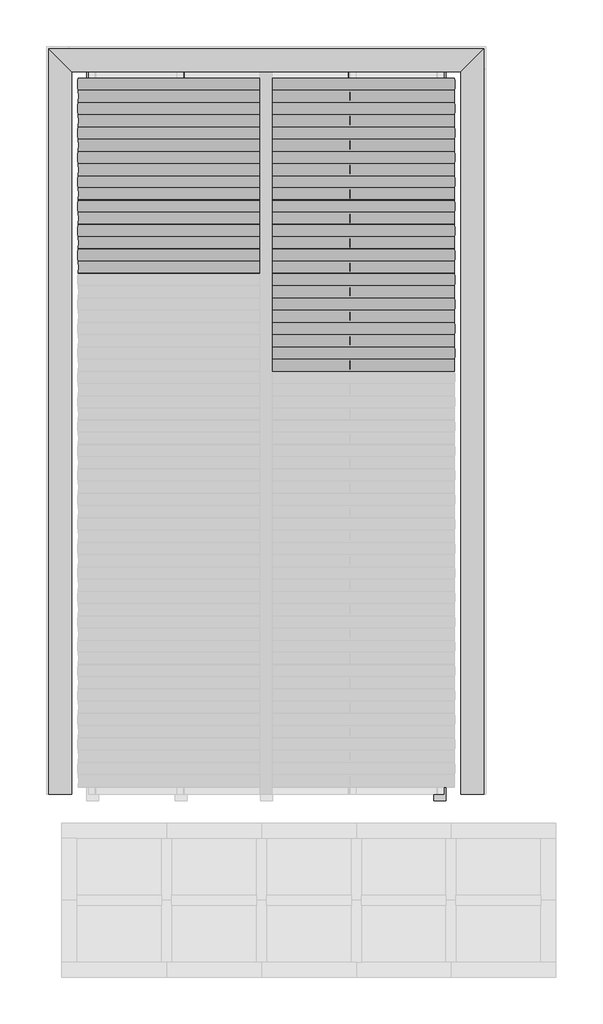
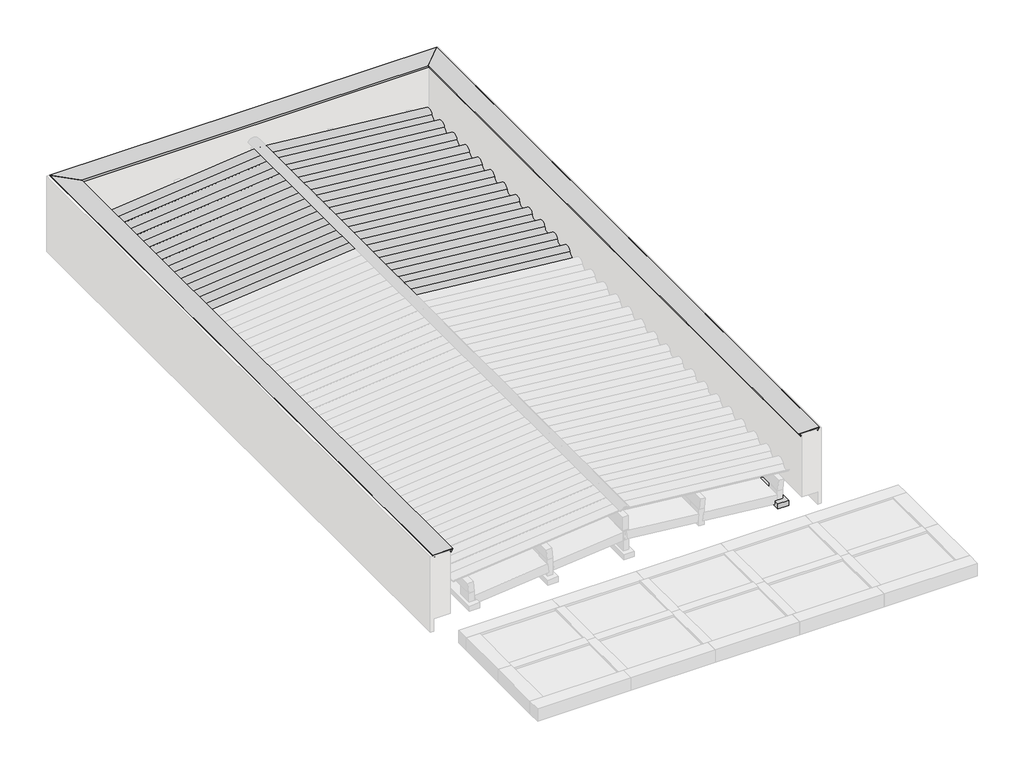
# One storey, part 3 of 3: 33 beams, 12 columns, 1 proxy.
"""IFC4 building model written with IfcOpenShell, lengths in millimetres."""

import ifcopenshell
import ifcopenshell.guid

model = None  # the IFC model being written
_history = None  # IfcOwnerHistory: only IFC2X3 demands one
_inside = {}  # id of a spatial element -> (the spatial element, [elements in it])
_under = {}  # id of a project, library or spatial element -> (it, [spatial elements below it])
_declared = {}  # id of a project -> (the project, [libraries it declares])
_typed = {}  # id of a type object -> (the type object, [elements of that type])
_made_of = {}  # id of a material, layer set ... -> (it, [elements and type objects made of it])


def new_model(schema):
    """Start an empty IFC model of exactly this schema.

    Asked for "IFC4X3", IfcOpenShell would pick the latest addendum, in which some entities
    have other attributes; the version numbers below select the first issue.
    IFC2X3 requires an IfcOwnerHistory on every rooted entity: one is made here for all.
    """
    global model, _history
    if schema == "IFC4X3":
        model = ifcopenshell.file(schema_version=(4, 3, 0, 0))
    else:
        model = ifcopenshell.file(schema=schema)
    _inside.clear()
    _under.clear()
    _declared.clear()
    _typed.clear()
    _made_of.clear()
    _history = None
    if model.schema == "IFC2X3":
        org = make("IfcOrganization", Name="unknown")
        user = make(
            "IfcPersonAndOrganization",
            ThePerson=make("IfcPerson", FamilyName="unknown"),
            TheOrganization=org,
        )
        app = make(
            "IfcApplication",
            ApplicationDeveloper=org,
            Version="unknown",
            ApplicationFullName="unknown",
            ApplicationIdentifier="unknown",
        )
        _history = make(
            "IfcOwnerHistory",
            OwningUser=user,
            OwningApplication=app,
            ChangeAction="ADDED",
            CreationDate=0,
        )
    return model


def make(cls, **values):
    """One entity of the class cls with the attributes given. An attribute that is None is left unset."""
    return model.create_entity(
        cls, **{name: value for name, value in values.items() if value is not None}
    )


def rooted(cls, **values):
    """An entity with a GlobalId (a new one), such as an element, a storey or a relation."""
    return make(cls, GlobalId=ifcopenshell.guid.new(), OwnerHistory=_history, **values)


def si_unit(unit_type, name, prefix=None):
    """IfcSIUnit, for example si_unit("LENGTHUNIT", "METRE", prefix="MILLI")."""
    return make("IfcSIUnit", UnitType=unit_type, Prefix=prefix, Name=name)


def assignment(units):
    """IfcUnitAssignment: the units of a project."""
    return None if units is None else make("IfcUnitAssignment", Units=units)


def point(xyz):
    """IfcCartesianPoint."""
    return None if xyz is None else make("IfcCartesianPoint", Coordinates=xyz)


def direction(xyz):
    """IfcDirection."""
    return None if xyz is None else make("IfcDirection", DirectionRatios=xyz)


def frame(location, z_axis=None, x_axis=None):
    """IfcAxis2Placement3D, a coordinate frame: its origin and axes. An axis left out is left unset."""
    return make(
        "IfcAxis2Placement3D",
        Location=point(location),
        Axis=direction(z_axis),
        RefDirection=direction(x_axis),
    )


def frame_2d(location, x_axis=None):
    """IfcAxis2Placement2D, a coordinate frame in the plane: its origin and x axis."""
    return make(
        "IfcAxis2Placement2D", Location=point(location), RefDirection=direction(x_axis)
    )


def origin():
    """The frame at (0, 0, 0) with its axes left unset."""
    return frame((0.0, 0.0, 0.0))


def place(relative_to, where):
    """IfcLocalPlacement: puts the frame where relative to a parent placement (None: the world)."""
    return make(
        "IfcLocalPlacement", PlacementRelTo=relative_to, RelativePlacement=where
    )


def context(
    kind, dimensions, precision=None, world=None, true_north=None, identifier=None
):
    """IfcGeometricRepresentationContext, for example the 3D "Model" context."""
    return make(
        "IfcGeometricRepresentationContext",
        ContextIdentifier=identifier,
        ContextType=kind,
        CoordinateSpaceDimension=dimensions,
        Precision=precision,
        WorldCoordinateSystem=world,
        TrueNorth=true_north,
    )


def project(units=None, contexts=None):
    """IfcProject with its units and contexts."""
    return rooted(
        "IfcProject",
        Name="project",
        RepresentationContexts=contexts,
        UnitsInContext=assignment(units),
    )


def spatial(cls, under=None, at=None, **own):
    """A site, building, storey or space (cls), placed at a placement, below another one or the project."""
    s = rooted(cls, ObjectPlacement=at, **own)
    if under is not None:
        _under.setdefault(under.id(), (under, []))[1].append(s)
    return s


def polyline(points):
    """IfcPolyline through the points."""
    return make("IfcPolyline", Points=[point(p) for p in points])


def circle_curve(where, radius):
    """IfcCircle in the frame where."""
    return make("IfcCircle", Position=where, Radius=radius)


def trimmed(basis, trim1, trim2, sense, master):
    """IfcTrimmedCurve: the piece of a basis curve between two trims."""
    return make(
        "IfcTrimmedCurve",
        BasisCurve=basis,
        Trim1=trim1,
        Trim2=trim2,
        SenseAgreement=sense,
        MasterRepresentation=master,
    )


def segment(curve, same_sense, transition):
    """IfcCompositeCurveSegment."""
    return make(
        "IfcCompositeCurveSegment",
        Transition=transition,
        SameSense=same_sense,
        ParentCurve=curve,
    )


def composite_curve(segments, self_intersect=None):
    """IfcCompositeCurve: segments joined end to end."""
    return make("IfcCompositeCurve", Segments=segments, SelfIntersect=self_intersect)


def outline(outer, holes=None, kind="AREA"):
    """IfcArbitraryClosedProfileDef: a profile drawn as a closed curve; with holes, ...WithVoids."""
    if holes is None:
        return make("IfcArbitraryClosedProfileDef", ProfileType=kind, OuterCurve=outer)
    return make(
        "IfcArbitraryProfileDefWithVoids",
        ProfileType=kind,
        OuterCurve=outer,
        InnerCurves=holes,
    )


def extrude(swept, where, along, depth):
    """IfcExtrudedAreaSolid: the profile swept, set in the frame where, extruded along a direction by depth."""
    return make(
        "IfcExtrudedAreaSolid",
        SweptArea=swept,
        Position=where,
        ExtrudedDirection=direction(along),
        Depth=depth,
    )


def faces_of(points, faces, orient=None, outer=None):
    """IfcFace entities. A face is a list of loops; a loop is a list of indices into points, from 0.

    orient and outer hold one flag for each loop. By default every Orientation is true, the
    first loop of a face is its IfcFaceOuterBound and the others are IfcFaceBound.
    """
    made = []
    for i, loops in enumerate(faces):
        bounds = []
        for j, loop in enumerate(loops):
            is_outer = j == 0 if outer is None else outer[i][j]
            bounds.append(
                make(
                    "IfcFaceOuterBound" if is_outer else "IfcFaceBound",
                    Bound=make("IfcPolyLoop", Polygon=[points[k] for k in loop]),
                    Orientation=True if orient is None else orient[i][j],
                )
            )
        made.append(make("IfcFace", Bounds=bounds))
    return made


def faceted_brep(points, faces, orient=None, outer=None, voids=None):
    """IfcFacetedBrep: a solid bounded by flat faces; with voids (closed shells), ...WithVoids."""
    shared = [point(p) for p in points]
    hull = make("IfcClosedShell", CfsFaces=faces_of(shared, faces, orient, outer))
    if voids is None:
        return make("IfcFacetedBrep", Outer=hull)
    return make(
        "IfcFacetedBrepWithVoids",
        Outer=hull,
        Voids=[
            make(cls, CfsFaces=faces_of(shared, fs, o, b)) for cls, fs, o, b in voids
        ],
    )


def shape(context_of_items, identifier, shape_type, items):
    """IfcShapeRepresentation: the items that make up one representation, for example the "Body"."""
    return make(
        "IfcShapeRepresentation",
        ContextOfItems=context_of_items,
        RepresentationIdentifier=identifier,
        RepresentationType=shape_type,
        Items=items,
    )


def source(mapping_origin, context_of_items, identifier, shape_type, items):
    """IfcRepresentationMap: a shape defined once, which mapped items show again and again."""
    return make(
        "IfcRepresentationMap",
        MappingOrigin=mapping_origin,
        MappedRepresentation=shape(context_of_items, identifier, shape_type, items),
    )


def transform(
    local_origin,
    x_axis=None,
    y_axis=None,
    z_axis=None,
    scale=None,
    scale2=None,
    scale3=None,
    uniform=True,
):
    """IfcCartesianTransformationOperator3D, or its non-uniform kind. x_axis, y_axis, z_axis: its Axis1, 2, 3."""
    if uniform:
        return make(
            "IfcCartesianTransformationOperator3D",
            Axis1=direction(x_axis),
            Axis2=direction(y_axis),
            LocalOrigin=point(local_origin),
            Scale=scale,
            Axis3=direction(z_axis),
        )
    return make(
        "IfcCartesianTransformationOperator3DnonUniform",
        Axis1=direction(x_axis),
        Axis2=direction(y_axis),
        LocalOrigin=point(local_origin),
        Scale=scale,
        Axis3=direction(z_axis),
        Scale2=scale2,
        Scale3=scale3,
    )


def mapped(mapping_source, mapping_target):
    """IfcMappedItem: shows the shape of a source again, moved by a transform."""
    return make(
        "IfcMappedItem", MappingSource=mapping_source, MappingTarget=mapping_target
    )


def made_of(thing, what):
    """Note that an element or type object is made of a material, layer set ...; save() writes the relation."""
    if what is not None:
        _made_of.setdefault(what.id(), (what, []))[1].append(thing)
    return thing


def element(
    cls,
    number,
    at=None,
    inside=None,
    cuts=None,
    type_object=None,
    material=None,
    context=None,
    identifier="Body",
    shape_type=None,
    held_by="IfcProductDefinitionShape",
    body=None,
    shapes=None,
    **own,
):
    """One element of the class cls, such as IfcWall. Its Tag is "e" and its number.

    at: its placement. inside: the storey or other place that contains it. cuts: it is an
    opening in that element (IfcRelVoidsElement). A single representation is given by context,
    identifier, shape_type and body (its items); several are given by shapes. held_by: the class
    of the entity that holds the representations. save() writes the other relations.
    """
    e = rooted(cls, Tag="e%d" % number, ObjectPlacement=at, **own)
    if body is not None:
        shapes = [shape(context, identifier, shape_type, body)]
    if shapes is not None:
        e.Representation = make(held_by, Representations=shapes)
    if inside is not None:
        _inside.setdefault(inside.id(), (inside, []))[1].append(e)
    if cuts is not None:
        rooted(
            "IfcRelVoidsElement", RelatingBuildingElement=cuts, RelatedOpeningElement=e
        )
    if type_object is not None:
        _typed.setdefault(type_object.id(), (type_object, []))[1].append(e)
    return made_of(e, material)


def aggregate(whole, parts):
    """IfcRelAggregates: a whole, such as a stair, and the parts it consists of."""
    return rooted("IfcRelAggregates", RelatingObject=whole, RelatedObjects=parts)


def save(model, path):
    """Write the relations noted so far, then the file.

    IfcRelAggregates (storeys below a building ...), IfcRelContainedInSpatialStructure (elements
    in a storey), IfcRelDefinesByType, IfcRelAssociatesMaterial and IfcRelDeclares: one each for
    every whole, place, type object, material and project.
    """
    for whole, parts in _under.values():
        aggregate(whole, parts)
    for where, things in _inside.values():
        rooted(
            "IfcRelContainedInSpatialStructure",
            RelatedElements=things,
            RelatingStructure=where,
        )
    for kind, things in _typed.values():
        rooted("IfcRelDefinesByType", RelatedObjects=things, RelatingType=kind)
    for what, things in _made_of.values():
        rooted("IfcRelAssociatesMaterial", RelatedObjects=things, RelatingMaterial=what)
    for by, libraries in _declared.values():
        rooted("IfcRelDeclares", RelatingContext=by, RelatedDefinitions=libraries)
    model.write(path)


def column_1cffec27(model_context):
    return source(origin(), model_context, "Body", "SweptSolid", [
        extrude(outline(polyline([(30.0, 80.0), (30.0, -80.0), (-30.0, -80.0), (-30.0, 80.0), (30.0, 80.0)])), frame((0.0, 0.0, 3110.0), z_axis=(0.0, 0.0, 1.0), x_axis=(1.0, 0.0, 0.0)), (0.0, 0.0, 1.0), 238.0),
    ])


def column_35730ad5(model_context):
    return source(origin(), model_context, "Body", "SweptSolid", [
        extrude(outline(polyline([(30.0, 80.0), (30.0, -80.0), (-30.0, -80.0), (-30.0, 80.0), (30.0, 80.0)])), frame((0.0, 0.0, 3110.0), z_axis=(0.0, 0.0, 1.0), x_axis=(1.0, 0.0, 0.0)), (0.0, 0.0, 1.0), 197.9),
    ])


def column_00c463e4(model_context):
    return source(origin(), model_context, "Body", "SweptSolid", [
        extrude(outline(polyline([(30.0, 80.0), (30.0, -80.0), (-30.0, -80.0), (-30.0, 80.0), (30.0, 80.0)])), frame((0.0, 0.0, 3110.0), z_axis=(0.0, 0.0, 1.0), x_axis=(1.0, 0.0, 0.0)), (0.0, 0.0, 1.0), 109.8),
    ])


model = new_model("IFC4")

# Units and contexts
model_context = context("Model", 3, world=origin())
ifc_project = project(units=[si_unit("LENGTHUNIT", "METRE", prefix="MILLI")], contexts=[model_context])

# Site, building, storey
site = spatial("IfcSite", under=ifc_project)
building = spatial("IfcBuilding", under=site)
storey = spatial("IfcBuildingStorey", under=building, Name="COB. GARAGEM", Elevation=3050.0)

# Beams
placement = place(None, origin())
element("IfcBeam", 1, ObjectType="Madeira de lei : Berço 6x12cm", at=placement, inside=storey, context=model_context, shape_type="SweptSolid", body=[
    extrude(outline(polyline([(-9620.281307, 6423.9300153), (-9500.281307, 6423.9300153), (-9500.281307, 4423.9300153), (-9620.281307, 4423.9300153), (-9620.281307, 6423.9300153)])), frame((0.0, 0.0, 3050.0), z_axis=(0.0, 0.0, 1.0), x_axis=(1.0, 0.0, 0.0)), (0.0, 0.0, 1.0), 60.0),
])
element("IfcBeam", 2, ObjectType="Madeira de lei : Berço 6x12cm", at=placement, inside=storey, context=model_context, shape_type="SweptSolid", body=[
    extrude(outline(polyline([(-9620.281307, 7083.9300153), (-9500.281307, 7083.9300153), (-9500.281307, 6423.9300153), (-9620.281307, 6423.9300153), (-9620.281307, 7083.9300153)])), frame((0.0, 0.0, 3050.0), z_axis=(0.0, 0.0, 1.0), x_axis=(1.0, 0.0, 0.0)), (0.0, 0.0, 1.0), 60.0),
])
element("IfcBeam", 3, ObjectType="Madeira de lei : Berço 6x12cm", at=placement, inside=storey, context=model_context, shape_type="SweptSolid", body=[
    extrude(outline(polyline([(-8767.0824227, 6423.9300153), (-8647.0824227, 6423.9300153), (-8647.0824227, 4423.9300153), (-8767.0824227, 4423.9300153), (-8767.0824227, 6423.9300153)])), frame((0.0, 0.0, 3050.0), z_axis=(0.0, 0.0, 1.0), x_axis=(1.0, 0.0, 0.0)), (0.0, 0.0, 1.0), 60.0),
])
element("IfcBeam", 4, ObjectType="Madeira de lei : Berço 6x12cm", at=placement, inside=storey, context=model_context, shape_type="SweptSolid", body=[
    extrude(outline(polyline([(-8767.0824227, 7083.9300153), (-8647.0824227, 7083.9300153), (-8647.0824227, 6423.9300153), (-8767.0824227, 6423.9300153), (-8767.0824227, 7083.9300153)])), frame((0.0, 0.0, 3050.0), z_axis=(0.0, 0.0, 1.0), x_axis=(1.0, 0.0, 0.0)), (0.0, 0.0, 1.0), 60.0),
])
element("IfcBeam", 5, ObjectType="Madeira de lei : Berço 6x12cm", at=placement, inside=storey, context=model_context, shape_type="SweptSolid", body=[
    extrude(outline(polyline([(-7884.0324227, 4423.9300153), (-7764.0324227, 4423.9300153), (-7764.0324227, 2423.9300153), (-7884.0324227, 2423.9300153), (-7884.0324227, 4423.9300153)])), frame((0.0, 0.0, 3050.0), z_axis=(0.0, 0.0, 1.0), x_axis=(1.0, 0.0, 0.0)), (0.0, 0.0, 1.0), 60.0),
])
element("IfcBeam", 6, ObjectType="Madeira de lei : Berço 6x12cm", at=placement, inside=storey, context=model_context, shape_type="SweptSolid", body=[
    extrude(outline(polyline([(-7884.0324227, 6423.9300153), (-7764.0324227, 6423.9300153), (-7764.0324227, 4423.9300153), (-7884.0324227, 4423.9300153), (-7884.0324227, 6423.9300153)])), frame((0.0, 0.0, 3050.0), z_axis=(0.0, 0.0, 1.0), x_axis=(1.0, 0.0, 0.0)), (0.0, 0.0, 1.0), 60.0),
])
element("IfcBeam", 7, ObjectType="Madeira de lei : Berço 6x12cm", at=placement, inside=storey, context=model_context, shape_type="SweptSolid", body=[
    extrude(outline(polyline([(-7884.0324227, 2423.9300153), (-7764.0324227, 2423.9300153), (-7764.0324227, 423.9300153), (-7884.0324227, 423.9300153), (-7884.0324227, 2423.9300153)])), frame((0.0, 0.0, 3050.0), z_axis=(0.0, 0.0, 1.0), x_axis=(1.0, 0.0, 0.0)), (0.0, 0.0, 1.0), 60.0),
])
element("IfcBeam", 8, ObjectType="Madeira de lei : Berço 6x12cm", at=placement, inside=storey, context=model_context, shape_type="SweptSolid", body=[
    extrude(outline(polyline([(-7884.0324227, 7083.9300153), (-7764.0324227, 7083.9300153), (-7764.0324227, 6423.9300153), (-7884.0324227, 6423.9300153), (-7884.0324227, 7083.9300153)])), frame((0.0, 0.0, 3050.0), z_axis=(0.0, 0.0, 1.0), x_axis=(1.0, 0.0, 0.0)), (0.0, 0.0, 1.0), 60.0),
])
element("IfcBeam", 9, ObjectType="Madeira de lei : Berço 6x12cm", at=placement, inside=storey, context=model_context, shape_type="SweptSolid", body=[
    extrude(outline(polyline([(-7884.0324227, 423.9300153), (-7764.0324227, 423.9300153), (-7764.0324227, -236.0699847), (-7884.0324227, -236.0699847), (-7884.0324227, 423.9300153)])), frame((0.0, 0.0, 3050.0), z_axis=(0.0, 0.0, 1.0), x_axis=(1.0, 0.0, 0.0)), (0.0, 0.0, 1.0), 60.0),
])
element("IfcBeam", 10, ObjectType="Madeira de lei : Berço 6x12cm", at=placement, inside=storey, context=model_context, shape_type="SweptSolid", body=[
    extrude(outline(polyline([(-10473.4801913, 6423.9300153), (-10353.4801913, 6423.9300153), (-10353.4801913, 4423.9300153), (-10473.4801913, 4423.9300153), (-10473.4801913, 6423.9300153)])), frame((0.0, 0.0, 3050.0), z_axis=(0.0, 0.0, 1.0), x_axis=(1.0, 0.0, 0.0)), (0.0, 0.0, 1.0), 60.0),
])
element("IfcBeam", 11, ObjectType="Madeira de lei : Berço 6x12cm", at=placement, inside=storey, context=model_context, shape_type="SweptSolid", body=[
    extrude(outline(polyline([(-10473.4801913, 7083.9300153), (-10353.4801913, 7083.9300153), (-10353.4801913, 6423.9300153), (-10473.4801913, 6423.9300153), (-10473.4801913, 7083.9300153)])), frame((0.0, 0.0, 3050.0), z_axis=(0.0, 0.0, 1.0), x_axis=(1.0, 0.0, 0.0)), (0.0, 0.0, 1.0), 60.0),
])
element("IfcBeam", 12, ObjectType="Madeira de lei : Berço 6x12cm", at=placement, inside=storey, context=model_context, shape_type="SweptSolid", body=[
    extrude(outline(polyline([(-11356.5301913, 6423.9300153), (-11236.5301913, 6423.9300153), (-11236.5301913, 4423.9300153), (-11356.5301913, 4423.9300153), (-11356.5301913, 6423.9300153)])), frame((0.0, 0.0, 3050.0), z_axis=(0.0, 0.0, 1.0), x_axis=(1.0, 0.0, 0.0)), (0.0, 0.0, 1.0), 60.0),
])
element("IfcBeam", 13, ObjectType="Madeira de lei : Berço 6x12cm", at=placement, inside=storey, context=model_context, shape_type="SweptSolid", body=[
    extrude(outline(polyline([(-11356.5301913, 7083.9300153), (-11236.5301913, 7083.9300153), (-11236.5301913, 6423.9300153), (-11356.5301913, 6423.9300153), (-11356.5301913, 7083.9300153)])), frame((0.0, 0.0, 3050.0), z_axis=(0.0, 0.0, 1.0), x_axis=(1.0, 0.0, 0.0)), (0.0, 0.0, 1.0), 60.0),
])
element("IfcBeam", 14, ObjectType="Telha Ondulada : Fibrocimento", at=placement, inside=storey, context=model_context, shape_type="SweptSolid", body=[
    extrude(outline(composite_curve([segment(trimmed(circle_curve(frame_2d((-58.7002979, -53.2060538)), 66.7939461), [point((-29.350149, 6.7939462))], [point((-29.350149, -113.2060538))], False, "CARTESIAN"), True, "CONTINUOUS"), segment(polyline([(-29.350149, -113.2060538), (-31.5472155, -108.7146288)]), True, "CONTINUOUS"), segment(trimmed(circle_curve(frame_2d((-58.7002979, -53.2060538)), 61.7939461), [point((-31.5472155, -108.7146288))], [point((-31.5472155, 2.3025211))], True, "CARTESIAN"), True, "CONTINUOUS"), segment(trimmed(circle_curve(frame_2d((0.0, 66.7939462)), 71.7939461), [point((-31.5472155, 2.3025211))], [point((-31.5472155, 131.2853712))], False, "CARTESIAN"), True, "CONTINUOUS"), segment(polyline([(-31.5472155, 131.2853712), (-29.350149, 126.7939462)]), True, "CONTINUOUS"), segment(trimmed(circle_curve(frame_2d((0.0, 66.7939462)), 66.7939461), [point((-29.350149, 126.7939462))], [point((-29.350149, 6.7939462))], True, "CARTESIAN"), True, "CONTINUOUS")], self_intersect=False)), frame((-11446.918865, 5163.326948, 3394.3067746), z_axis=(0.9950371902099892, 0.0, 0.09950371902099937), x_axis=(-0.09950371902099937, 0.0, 0.9950371902099892)), (0.0, 0.0, 1.0), 1886.8678854),
])
element("IfcBeam", 15, ObjectType="Telha Ondulada : Fibrocimento", at=placement, inside=storey, context=model_context, shape_type="SweptSolid", body=[
    extrude(outline(composite_curve([segment(trimmed(circle_curve(frame_2d((-58.7002979, -53.2060538)), 66.7939461), [point((-29.350149, 6.7939462))], [point((-29.350149, -113.2060538))], False, "CARTESIAN"), True, "CONTINUOUS"), segment(polyline([(-29.350149, -113.2060538), (-31.5472155, -108.7146288)]), True, "CONTINUOUS"), segment(trimmed(circle_curve(frame_2d((-58.7002979, -53.2060538)), 61.7939461), [point((-31.5472155, -108.7146288))], [point((-31.5472155, 2.3025211))], True, "CARTESIAN"), True, "CONTINUOUS"), segment(trimmed(circle_curve(frame_2d((0.0, 66.7939462)), 71.7939461), [point((-31.5472155, 2.3025211))], [point((-31.5472155, 131.2853712))], False, "CARTESIAN"), True, "CONTINUOUS"), segment(polyline([(-31.5472155, 131.2853712), (-29.350149, 126.7939462)]), True, "CONTINUOUS"), segment(trimmed(circle_curve(frame_2d((0.0, 66.7939462)), 66.7939461), [point((-29.350149, 126.7939462))], [point((-29.350149, 6.7939462))], True, "CARTESIAN"), True, "CONTINUOUS")], self_intersect=False)), frame((-11446.918865, 5407.826948, 3394.3067746), z_axis=(0.9950371902099892, 0.0, 0.09950371902099972), x_axis=(-0.09950371902099972, 0.0, 0.9950371902099892)), (0.0, 0.0, 1.0), 1886.8678854),
])
element("IfcBeam", 16, ObjectType="Telha Ondulada : Fibrocimento", at=placement, inside=storey, context=model_context, shape_type="SweptSolid", body=[
    extrude(outline(composite_curve([segment(trimmed(circle_curve(frame_2d((-58.7002979, -53.2060538)), 66.7939461), [point((-29.350149, 6.7939462))], [point((-29.350149, -113.2060538))], False, "CARTESIAN"), True, "CONTINUOUS"), segment(polyline([(-29.350149, -113.2060538), (-31.5472155, -108.7146288)]), True, "CONTINUOUS"), segment(trimmed(circle_curve(frame_2d((-58.7002979, -53.2060538)), 61.7939461), [point((-31.5472155, -108.7146288))], [point((-31.5472155, 2.3025211))], True, "CARTESIAN"), True, "CONTINUOUS"), segment(trimmed(circle_curve(frame_2d((0.0, 66.7939462)), 71.7939461), [point((-31.5472155, 2.3025211))], [point((-31.5472155, 131.2853712))], False, "CARTESIAN"), True, "CONTINUOUS"), segment(polyline([(-31.5472155, 131.2853712), (-29.350149, 126.7939462)]), True, "CONTINUOUS"), segment(trimmed(circle_curve(frame_2d((0.0, 66.7939462)), 66.7939461), [point((-29.350149, 126.7939462))], [point((-29.350149, 6.7939462))], True, "CARTESIAN"), True, "CONTINUOUS")], self_intersect=False)), frame((-11446.918865, 5652.326948, 3394.3067746), z_axis=(0.9950371902099892, 0.0, 0.09950371902099954), x_axis=(-0.09950371902099954, 0.0, 0.9950371902099892)), (0.0, 0.0, 1.0), 1886.8678854),
])
element("IfcBeam", 17, ObjectType="Telha Ondulada : Fibrocimento", at=placement, inside=storey, context=model_context, shape_type="SweptSolid", body=[
    extrude(outline(composite_curve([segment(trimmed(circle_curve(frame_2d((-58.7002979, -53.2060538)), 66.7939461), [point((-29.350149, 6.7939462))], [point((-29.350149, -113.2060538))], False, "CARTESIAN"), True, "CONTINUOUS"), segment(polyline([(-29.350149, -113.2060538), (-31.5472155, -108.7146288)]), True, "CONTINUOUS"), segment(trimmed(circle_curve(frame_2d((-58.7002979, -53.2060538)), 61.7939461), [point((-31.5472155, -108.7146288))], [point((-31.5472155, 2.3025211))], True, "CARTESIAN"), True, "CONTINUOUS"), segment(trimmed(circle_curve(frame_2d((0.0, 66.7939462)), 71.7939461), [point((-31.5472155, 2.3025211))], [point((-31.5472155, 131.2853712))], False, "CARTESIAN"), True, "CONTINUOUS"), segment(polyline([(-31.5472155, 131.2853712), (-29.350149, 126.7939462)]), True, "CONTINUOUS"), segment(trimmed(circle_curve(frame_2d((0.0, 66.7939462)), 66.7939461), [point((-29.350149, 126.7939462))], [point((-29.350149, 6.7939462))], True, "CARTESIAN"), True, "CONTINUOUS")], self_intersect=False)), frame((-11446.918865, 5896.826948, 3394.3067746), z_axis=(0.9950371902099892, 0.0, 0.09950371902099932), x_axis=(-0.09950371902099932, 0.0, 0.9950371902099892)), (0.0, 0.0, 1.0), 1886.8678854),
])
element("IfcBeam", 18, ObjectType="Telha Ondulada : Fibrocimento", at=placement, inside=storey, context=model_context, shape_type="SweptSolid", body=[
    extrude(outline(composite_curve([segment(trimmed(circle_curve(frame_2d((-58.7002979, -53.2060538)), 66.7939461), [point((-29.350149, 6.7939462))], [point((-29.350149, -113.2060538))], False, "CARTESIAN"), True, "CONTINUOUS"), segment(polyline([(-29.350149, -113.2060538), (-31.5472155, -108.7146288)]), True, "CONTINUOUS"), segment(trimmed(circle_curve(frame_2d((-58.7002979, -53.2060538)), 61.7939461), [point((-31.5472155, -108.7146288))], [point((-31.5472155, 2.3025211))], True, "CARTESIAN"), True, "CONTINUOUS"), segment(trimmed(circle_curve(frame_2d((0.0, 66.7939462)), 71.7939461), [point((-31.5472155, 2.3025211))], [point((-31.5472155, 131.2853712))], False, "CARTESIAN"), True, "CONTINUOUS"), segment(polyline([(-31.5472155, 131.2853712), (-29.350149, 126.7939462)]), True, "CONTINUOUS"), segment(trimmed(circle_curve(frame_2d((0.0, 66.7939462)), 66.7939461), [point((-29.350149, 126.7939462))], [point((-29.350149, 6.7939462))], True, "CARTESIAN"), True, "CONTINUOUS")], self_intersect=False)), frame((-11446.918865, 6141.326948, 3394.3067746), z_axis=(0.9950371902099892, 0.0, 0.09950371902099943), x_axis=(-0.09950371902099943, 0.0, 0.9950371902099892)), (0.0, 0.0, 1.0), 1886.8678854),
])
element("IfcBeam", 19, ObjectType="Telha Ondulada : Fibrocimento", at=placement, inside=storey, context=model_context, shape_type="SweptSolid", body=[
    extrude(outline(composite_curve([segment(trimmed(circle_curve(frame_2d((-58.7002979, -53.2060538)), 66.7939461), [point((-29.350149, 6.7939462))], [point((-29.350149, -113.2060538))], False, "CARTESIAN"), True, "CONTINUOUS"), segment(polyline([(-29.350149, -113.2060538), (-31.5472155, -108.7146288)]), True, "CONTINUOUS"), segment(trimmed(circle_curve(frame_2d((-58.7002979, -53.2060538)), 61.7939461), [point((-31.5472155, -108.7146288))], [point((-31.5472155, 2.3025211))], True, "CARTESIAN"), True, "CONTINUOUS"), segment(trimmed(circle_curve(frame_2d((0.0, 66.7939462)), 71.7939461), [point((-31.5472155, 2.3025211))], [point((-31.5472155, 131.2853712))], False, "CARTESIAN"), True, "CONTINUOUS"), segment(polyline([(-31.5472155, 131.2853712), (-29.350149, 126.7939462)]), True, "CONTINUOUS"), segment(trimmed(circle_curve(frame_2d((0.0, 66.7939462)), 66.7939461), [point((-29.350149, 126.7939462))], [point((-29.350149, 6.7939462))], True, "CARTESIAN"), True, "CONTINUOUS")], self_intersect=False)), frame((-11446.918865, 6385.826948, 3394.3067746), z_axis=(0.9950371902099892, 0.0, 0.09950371902099919), x_axis=(-0.09950371902099919, 0.0, 0.9950371902099892)), (0.0, 0.0, 1.0), 1886.8678854),
])
element("IfcBeam", 20, ObjectType="Telha Ondulada : Fibrocimento", at=placement, inside=storey, context=model_context, shape_type="SweptSolid", body=[
    extrude(outline(composite_curve([segment(trimmed(circle_curve(frame_2d((-58.7002979, -53.2060538)), 66.7939461), [point((-29.350149, 6.7939462))], [point((-29.350149, -113.2060538))], False, "CARTESIAN"), True, "CONTINUOUS"), segment(polyline([(-29.350149, -113.2060538), (-31.5472155, -108.7146288)]), True, "CONTINUOUS"), segment(trimmed(circle_curve(frame_2d((-58.7002979, -53.2060538)), 61.7939461), [point((-31.5472155, -108.7146288))], [point((-31.5472155, 2.3025211))], True, "CARTESIAN"), True, "CONTINUOUS"), segment(trimmed(circle_curve(frame_2d((0.0, 66.7939462)), 71.7939461), [point((-31.5472155, 2.3025211))], [point((-31.5472155, 131.2853712))], False, "CARTESIAN"), True, "CONTINUOUS"), segment(polyline([(-31.5472155, 131.2853712), (-29.350149, 126.7939462)]), True, "CONTINUOUS"), segment(trimmed(circle_curve(frame_2d((0.0, 66.7939462)), 66.7939461), [point((-29.350149, 126.7939462))], [point((-29.350149, 6.7939462))], True, "CARTESIAN"), True, "CONTINUOUS")], self_intersect=False)), frame((-11446.918865, 6630.326948, 3394.3067746), z_axis=(0.9950371902099892, 0.0, 0.09950371902099925), x_axis=(-0.09950371902099925, 0.0, 0.9950371902099892)), (0.0, 0.0, 1.0), 1886.8678854),
])
element("IfcBeam", 21, ObjectType="Telha Ondulada : Fibrocimento", at=placement, inside=storey, context=model_context, shape_type="SweptSolid", body=[
    extrude(outline(composite_curve([segment(trimmed(circle_curve(frame_2d((-58.7002979, -53.2060538)), 66.7939461), [point((-29.350149, 6.7939462))], [point((-29.350149, -113.2060538))], False, "CARTESIAN"), True, "CONTINUOUS"), segment(polyline([(-29.350149, -113.2060538), (-31.5472155, -108.7146288)]), True, "CONTINUOUS"), segment(trimmed(circle_curve(frame_2d((-58.7002979, -53.2060538)), 61.7939461), [point((-31.5472155, -108.7146288))], [point((-31.5472155, 2.3025211))], True, "CARTESIAN"), True, "CONTINUOUS"), segment(trimmed(circle_curve(frame_2d((0.0, 66.7939462)), 71.7939461), [point((-31.5472155, 2.3025211))], [point((-31.5472155, 131.2853712))], False, "CARTESIAN"), True, "CONTINUOUS"), segment(polyline([(-31.5472155, 131.2853712), (-29.350149, 126.7939462)]), True, "CONTINUOUS"), segment(trimmed(circle_curve(frame_2d((0.0, 66.7939462)), 66.7939461), [point((-29.350149, 126.7939462))], [point((-29.350149, 6.7939462))], True, "CARTESIAN"), True, "CONTINUOUS")], self_intersect=False)), frame((-11446.918865, 6874.826948, 3394.3067746), z_axis=(0.9950371902099892, 0.0, 0.09950371902099937), x_axis=(-0.09950371902099937, 0.0, 0.9950371902099892)), (0.0, 0.0, 1.0), 1886.8678854),
])
element("IfcBeam", 22, ObjectType="Telha Ondulada : Fibrocimento", at=placement, inside=storey, context=model_context, shape_type="SweptSolid", body=[
    extrude(outline(composite_curve([segment(trimmed(circle_curve(frame_2d((0.0, 66.7939462)), 66.7939461), [point((29.350149, 6.7939462))], [point((29.350149, 126.7939462))], True, "CARTESIAN"), True, "CONTINUOUS"), segment(polyline([(29.350149, 126.7939462), (31.5472155, 131.2853712)]), True, "CONTINUOUS"), segment(trimmed(circle_curve(frame_2d((0.0, 66.7939462)), 71.7939461), [point((31.5472155, 131.2853712))], [point((31.5472155, 2.3025211))], False, "CARTESIAN"), True, "CONTINUOUS"), segment(trimmed(circle_curve(frame_2d((58.7002979, -53.2060538)), 61.7939461), [point((31.5472155, 2.3025211))], [point((31.5472155, -108.7146288))], True, "CARTESIAN"), True, "CONTINUOUS"), segment(polyline([(31.5472155, -108.7146288), (29.350149, -113.2060538)]), True, "CONTINUOUS"), segment(trimmed(circle_curve(frame_2d((58.7002979, -53.2060538)), 66.7939461), [point((29.350149, -113.2060538))], [point((29.350149, 6.7939462))], False, "CARTESIAN"), True, "CONTINUOUS")], self_intersect=False)), frame((-7673.6437489, 4185.326948, 3394.3067746), z_axis=(-0.9950371902099892, 0.0, 0.09950371902099965), x_axis=(-0.09950371902099965, 0.0, -0.9950371902099892)), (0.0, 0.0, 1.0), 1886.8678854),
])
element("IfcBeam", 23, ObjectType="Telha Ondulada : Fibrocimento", at=placement, inside=storey, context=model_context, shape_type="SweptSolid", body=[
    extrude(outline(composite_curve([segment(trimmed(circle_curve(frame_2d((0.0, 66.7939462)), 66.7939461), [point((29.350149, 6.7939462))], [point((29.350149, 126.7939462))], True, "CARTESIAN"), True, "CONTINUOUS"), segment(polyline([(29.350149, 126.7939462), (31.5472155, 131.2853712)]), True, "CONTINUOUS"), segment(trimmed(circle_curve(frame_2d((0.0, 66.7939462)), 71.7939461), [point((31.5472155, 131.2853712))], [point((31.5472155, 2.3025211))], False, "CARTESIAN"), True, "CONTINUOUS"), segment(trimmed(circle_curve(frame_2d((58.7002979, -53.2060538)), 61.7939461), [point((31.5472155, 2.3025211))], [point((31.5472155, -108.7146288))], True, "CARTESIAN"), True, "CONTINUOUS"), segment(polyline([(31.5472155, -108.7146288), (29.350149, -113.2060538)]), True, "CONTINUOUS"), segment(trimmed(circle_curve(frame_2d((58.7002979, -53.2060538)), 66.7939461), [point((29.350149, -113.2060538))], [point((29.350149, 6.7939462))], False, "CARTESIAN"), True, "CONTINUOUS")], self_intersect=False)), frame((-7673.6437489, 4429.826948, 3394.3067746), z_axis=(-0.9950371902099892, 0.0, 0.09950371902099965), x_axis=(-0.09950371902099965, 0.0, -0.9950371902099892)), (0.0, 0.0, 1.0), 1886.8678854),
])
element("IfcBeam", 24, ObjectType="Telha Ondulada : Fibrocimento", at=placement, inside=storey, context=model_context, shape_type="SweptSolid", body=[
    extrude(outline(composite_curve([segment(trimmed(circle_curve(frame_2d((0.0, 66.7939462)), 66.7939461), [point((29.350149, 6.7939462))], [point((29.350149, 126.7939462))], True, "CARTESIAN"), True, "CONTINUOUS"), segment(polyline([(29.350149, 126.7939462), (31.5472155, 131.2853712)]), True, "CONTINUOUS"), segment(trimmed(circle_curve(frame_2d((0.0, 66.7939462)), 71.7939461), [point((31.5472155, 131.2853712))], [point((31.5472155, 2.3025211))], False, "CARTESIAN"), True, "CONTINUOUS"), segment(trimmed(circle_curve(frame_2d((58.7002979, -53.2060538)), 61.7939461), [point((31.5472155, 2.3025211))], [point((31.5472155, -108.7146288))], True, "CARTESIAN"), True, "CONTINUOUS"), segment(polyline([(31.5472155, -108.7146288), (29.350149, -113.2060538)]), True, "CONTINUOUS"), segment(trimmed(circle_curve(frame_2d((58.7002979, -53.2060538)), 66.7939461), [point((29.350149, -113.2060538))], [point((29.350149, 6.7939462))], False, "CARTESIAN"), True, "CONTINUOUS")], self_intersect=False)), frame((-7673.6437489, 4674.326948, 3394.3067746), z_axis=(-0.9950371902099892, 0.0, 0.09950371902099965), x_axis=(-0.09950371902099965, 0.0, -0.9950371902099892)), (0.0, 0.0, 1.0), 1886.8678854),
])
element("IfcBeam", 25, ObjectType="Telha Ondulada : Fibrocimento", at=placement, inside=storey, context=model_context, shape_type="SweptSolid", body=[
    extrude(outline(composite_curve([segment(trimmed(circle_curve(frame_2d((0.0, 66.7939462)), 66.7939461), [point((29.350149, 6.7939462))], [point((29.350149, 126.7939462))], True, "CARTESIAN"), True, "CONTINUOUS"), segment(polyline([(29.350149, 126.7939462), (31.5472155, 131.2853712)]), True, "CONTINUOUS"), segment(trimmed(circle_curve(frame_2d((0.0, 66.7939462)), 71.7939461), [point((31.5472155, 131.2853712))], [point((31.5472155, 2.3025211))], False, "CARTESIAN"), True, "CONTINUOUS"), segment(trimmed(circle_curve(frame_2d((58.7002979, -53.2060538)), 61.7939461), [point((31.5472155, 2.3025211))], [point((31.5472155, -108.7146288))], True, "CARTESIAN"), True, "CONTINUOUS"), segment(polyline([(31.5472155, -108.7146288), (29.350149, -113.2060538)]), True, "CONTINUOUS"), segment(trimmed(circle_curve(frame_2d((58.7002979, -53.2060538)), 66.7939461), [point((29.350149, -113.2060538))], [point((29.350149, 6.7939462))], False, "CARTESIAN"), True, "CONTINUOUS")], self_intersect=False)), frame((-7673.6437489, 4918.826948, 3394.3067746), z_axis=(-0.9950371902099892, 0.0, 0.09950371902099965), x_axis=(-0.09950371902099965, 0.0, -0.9950371902099892)), (0.0, 0.0, 1.0), 1886.8678854),
])
element("IfcBeam", 26, ObjectType="Telha Ondulada : Fibrocimento", at=placement, inside=storey, context=model_context, shape_type="SweptSolid", body=[
    extrude(outline(composite_curve([segment(trimmed(circle_curve(frame_2d((0.0, 66.7939462)), 66.7939461), [point((29.350149, 6.7939462))], [point((29.350149, 126.7939462))], True, "CARTESIAN"), True, "CONTINUOUS"), segment(polyline([(29.350149, 126.7939462), (31.5472155, 131.2853712)]), True, "CONTINUOUS"), segment(trimmed(circle_curve(frame_2d((0.0, 66.7939462)), 71.7939461), [point((31.5472155, 131.2853712))], [point((31.5472155, 2.3025211))], False, "CARTESIAN"), True, "CONTINUOUS"), segment(trimmed(circle_curve(frame_2d((58.7002979, -53.2060538)), 61.7939461), [point((31.5472155, 2.3025211))], [point((31.5472155, -108.7146288))], True, "CARTESIAN"), True, "CONTINUOUS"), segment(polyline([(31.5472155, -108.7146288), (29.350149, -113.2060538)]), True, "CONTINUOUS"), segment(trimmed(circle_curve(frame_2d((58.7002979, -53.2060538)), 66.7939461), [point((29.350149, -113.2060538))], [point((29.350149, 6.7939462))], False, "CARTESIAN"), True, "CONTINUOUS")], self_intersect=False)), frame((-7673.6437489, 5163.326948, 3394.3067746), z_axis=(-0.9950371902099892, 0.0, 0.09950371902099965), x_axis=(-0.09950371902099965, 0.0, -0.9950371902099892)), (0.0, 0.0, 1.0), 1886.8678854),
])
element("IfcBeam", 27, ObjectType="Telha Ondulada : Fibrocimento", at=placement, inside=storey, context=model_context, shape_type="SweptSolid", body=[
    extrude(outline(composite_curve([segment(trimmed(circle_curve(frame_2d((0.0, 66.7939462)), 66.7939461), [point((29.350149, 6.7939462))], [point((29.350149, 126.7939462))], True, "CARTESIAN"), True, "CONTINUOUS"), segment(polyline([(29.350149, 126.7939462), (31.5472155, 131.2853712)]), True, "CONTINUOUS"), segment(trimmed(circle_curve(frame_2d((0.0, 66.7939462)), 71.7939461), [point((31.5472155, 131.2853712))], [point((31.5472155, 2.3025211))], False, "CARTESIAN"), True, "CONTINUOUS"), segment(trimmed(circle_curve(frame_2d((58.7002979, -53.2060538)), 61.7939461), [point((31.5472155, 2.3025211))], [point((31.5472155, -108.7146288))], True, "CARTESIAN"), True, "CONTINUOUS"), segment(polyline([(31.5472155, -108.7146288), (29.350149, -113.2060538)]), True, "CONTINUOUS"), segment(trimmed(circle_curve(frame_2d((58.7002979, -53.2060538)), 66.7939461), [point((29.350149, -113.2060538))], [point((29.350149, 6.7939462))], False, "CARTESIAN"), True, "CONTINUOUS")], self_intersect=False)), frame((-7673.6437489, 5407.826948, 3394.3067746), z_axis=(-0.9950371902099892, 0.0, 0.09950371902099965), x_axis=(-0.09950371902099965, 0.0, -0.9950371902099892)), (0.0, 0.0, 1.0), 1886.8678854),
])
element("IfcBeam", 28, ObjectType="Telha Ondulada : Fibrocimento", at=placement, inside=storey, context=model_context, shape_type="SweptSolid", body=[
    extrude(outline(composite_curve([segment(trimmed(circle_curve(frame_2d((0.0, 66.7939462)), 66.7939461), [point((29.350149, 6.7939462))], [point((29.350149, 126.7939462))], True, "CARTESIAN"), True, "CONTINUOUS"), segment(polyline([(29.350149, 126.7939462), (31.5472155, 131.2853712)]), True, "CONTINUOUS"), segment(trimmed(circle_curve(frame_2d((0.0, 66.7939462)), 71.7939461), [point((31.5472155, 131.2853712))], [point((31.5472155, 2.3025211))], False, "CARTESIAN"), True, "CONTINUOUS"), segment(trimmed(circle_curve(frame_2d((58.7002979, -53.2060538)), 61.7939461), [point((31.5472155, 2.3025211))], [point((31.5472155, -108.7146288))], True, "CARTESIAN"), True, "CONTINUOUS"), segment(polyline([(31.5472155, -108.7146288), (29.350149, -113.2060538)]), True, "CONTINUOUS"), segment(trimmed(circle_curve(frame_2d((58.7002979, -53.2060538)), 66.7939461), [point((29.350149, -113.2060538))], [point((29.350149, 6.7939462))], False, "CARTESIAN"), True, "CONTINUOUS")], self_intersect=False)), frame((-7673.6437489, 5652.326948, 3394.3067746), z_axis=(-0.9950371902099892, 0.0, 0.09950371902099965), x_axis=(-0.09950371902099965, 0.0, -0.9950371902099892)), (0.0, 0.0, 1.0), 1886.8678854),
])
element("IfcBeam", 29, ObjectType="Telha Ondulada : Fibrocimento", at=placement, inside=storey, context=model_context, shape_type="SweptSolid", body=[
    extrude(outline(composite_curve([segment(trimmed(circle_curve(frame_2d((0.0, 66.7939462)), 66.7939461), [point((29.350149, 6.7939462))], [point((29.350149, 126.7939462))], True, "CARTESIAN"), True, "CONTINUOUS"), segment(polyline([(29.350149, 126.7939462), (31.5472155, 131.2853712)]), True, "CONTINUOUS"), segment(trimmed(circle_curve(frame_2d((0.0, 66.7939462)), 71.7939461), [point((31.5472155, 131.2853712))], [point((31.5472155, 2.3025211))], False, "CARTESIAN"), True, "CONTINUOUS"), segment(trimmed(circle_curve(frame_2d((58.7002979, -53.2060538)), 61.7939461), [point((31.5472155, 2.3025211))], [point((31.5472155, -108.7146288))], True, "CARTESIAN"), True, "CONTINUOUS"), segment(polyline([(31.5472155, -108.7146288), (29.350149, -113.2060538)]), True, "CONTINUOUS"), segment(trimmed(circle_curve(frame_2d((58.7002979, -53.2060538)), 66.7939461), [point((29.350149, -113.2060538))], [point((29.350149, 6.7939462))], False, "CARTESIAN"), True, "CONTINUOUS")], self_intersect=False)), frame((-7673.6437489, 5896.826948, 3394.3067746), z_axis=(-0.9950371902099892, 0.0, 0.09950371902099965), x_axis=(-0.09950371902099965, 0.0, -0.9950371902099892)), (0.0, 0.0, 1.0), 1886.8678854),
])
element("IfcBeam", 30, ObjectType="Telha Ondulada : Fibrocimento", at=placement, inside=storey, context=model_context, shape_type="SweptSolid", body=[
    extrude(outline(composite_curve([segment(trimmed(circle_curve(frame_2d((0.0, 66.7939462)), 66.7939461), [point((29.350149, 6.7939462))], [point((29.350149, 126.7939462))], True, "CARTESIAN"), True, "CONTINUOUS"), segment(polyline([(29.350149, 126.7939462), (31.5472155, 131.2853712)]), True, "CONTINUOUS"), segment(trimmed(circle_curve(frame_2d((0.0, 66.7939462)), 71.7939461), [point((31.5472155, 131.2853712))], [point((31.5472155, 2.3025211))], False, "CARTESIAN"), True, "CONTINUOUS"), segment(trimmed(circle_curve(frame_2d((58.7002979, -53.2060538)), 61.7939461), [point((31.5472155, 2.3025211))], [point((31.5472155, -108.7146288))], True, "CARTESIAN"), True, "CONTINUOUS"), segment(polyline([(31.5472155, -108.7146288), (29.350149, -113.2060538)]), True, "CONTINUOUS"), segment(trimmed(circle_curve(frame_2d((58.7002979, -53.2060538)), 66.7939461), [point((29.350149, -113.2060538))], [point((29.350149, 6.7939462))], False, "CARTESIAN"), True, "CONTINUOUS")], self_intersect=False)), frame((-7673.6437489, 6141.326948, 3394.3067746), z_axis=(-0.9950371902099892, 0.0, 0.09950371902099965), x_axis=(-0.09950371902099965, 0.0, -0.9950371902099892)), (0.0, 0.0, 1.0), 1886.8678854),
])
element("IfcBeam", 31, ObjectType="Telha Ondulada : Fibrocimento", at=placement, inside=storey, context=model_context, shape_type="SweptSolid", body=[
    extrude(outline(composite_curve([segment(trimmed(circle_curve(frame_2d((0.0, 66.7939462)), 66.7939461), [point((29.350149, 6.7939462))], [point((29.350149, 126.7939462))], True, "CARTESIAN"), True, "CONTINUOUS"), segment(polyline([(29.350149, 126.7939462), (31.5472155, 131.2853712)]), True, "CONTINUOUS"), segment(trimmed(circle_curve(frame_2d((0.0, 66.7939462)), 71.7939461), [point((31.5472155, 131.2853712))], [point((31.5472155, 2.3025211))], False, "CARTESIAN"), True, "CONTINUOUS"), segment(trimmed(circle_curve(frame_2d((58.7002979, -53.2060538)), 61.7939461), [point((31.5472155, 2.3025211))], [point((31.5472155, -108.7146288))], True, "CARTESIAN"), True, "CONTINUOUS"), segment(polyline([(31.5472155, -108.7146288), (29.350149, -113.2060538)]), True, "CONTINUOUS"), segment(trimmed(circle_curve(frame_2d((58.7002979, -53.2060538)), 66.7939461), [point((29.350149, -113.2060538))], [point((29.350149, 6.7939462))], False, "CARTESIAN"), True, "CONTINUOUS")], self_intersect=False)), frame((-7673.6437489, 6385.826948, 3394.3067746), z_axis=(-0.9950371902099892, 0.0, 0.09950371902099965), x_axis=(-0.09950371902099965, 0.0, -0.9950371902099892)), (0.0, 0.0, 1.0), 1886.8678854),
])
element("IfcBeam", 32, ObjectType="Telha Ondulada : Fibrocimento", at=placement, inside=storey, context=model_context, shape_type="SweptSolid", body=[
    extrude(outline(composite_curve([segment(trimmed(circle_curve(frame_2d((0.0, 66.7939462)), 66.7939461), [point((29.350149, 6.7939462))], [point((29.350149, 126.7939462))], True, "CARTESIAN"), True, "CONTINUOUS"), segment(polyline([(29.350149, 126.7939462), (31.5472155, 131.2853712)]), True, "CONTINUOUS"), segment(trimmed(circle_curve(frame_2d((0.0, 66.7939462)), 71.7939461), [point((31.5472155, 131.2853712))], [point((31.5472155, 2.3025211))], False, "CARTESIAN"), True, "CONTINUOUS"), segment(trimmed(circle_curve(frame_2d((58.7002979, -53.2060538)), 61.7939461), [point((31.5472155, 2.3025211))], [point((31.5472155, -108.7146288))], True, "CARTESIAN"), True, "CONTINUOUS"), segment(polyline([(31.5472155, -108.7146288), (29.350149, -113.2060538)]), True, "CONTINUOUS"), segment(trimmed(circle_curve(frame_2d((58.7002979, -53.2060538)), 66.7939461), [point((29.350149, -113.2060538))], [point((29.350149, 6.7939462))], False, "CARTESIAN"), True, "CONTINUOUS")], self_intersect=False)), frame((-7673.6437489, 6630.326948, 3394.3067746), z_axis=(-0.9950371902099892, 0.0, 0.09950371902099965), x_axis=(-0.09950371902099965, 0.0, -0.9950371902099892)), (0.0, 0.0, 1.0), 1886.8678854),
])
element("IfcBeam", 33, ObjectType="Telha Ondulada : Fibrocimento", at=placement, inside=storey, context=model_context, shape_type="SweptSolid", body=[
    extrude(outline(composite_curve([segment(trimmed(circle_curve(frame_2d((0.0, 66.7939462)), 66.7939461), [point((29.350149, 6.7939462))], [point((29.350149, 126.7939462))], True, "CARTESIAN"), True, "CONTINUOUS"), segment(polyline([(29.350149, 126.7939462), (31.5472155, 131.2853712)]), True, "CONTINUOUS"), segment(trimmed(circle_curve(frame_2d((0.0, 66.7939462)), 71.7939461), [point((31.5472155, 131.2853712))], [point((31.5472155, 2.3025211))], False, "CARTESIAN"), True, "CONTINUOUS"), segment(trimmed(circle_curve(frame_2d((58.7002979, -53.2060538)), 61.7939461), [point((31.5472155, 2.3025211))], [point((31.5472155, -108.7146288))], True, "CARTESIAN"), True, "CONTINUOUS"), segment(polyline([(31.5472155, -108.7146288), (29.350149, -113.2060538)]), True, "CONTINUOUS"), segment(trimmed(circle_curve(frame_2d((58.7002979, -53.2060538)), 66.7939461), [point((29.350149, -113.2060538))], [point((29.350149, 6.7939462))], False, "CARTESIAN"), True, "CONTINUOUS")], self_intersect=False)), frame((-7673.6437489, 6874.826948, 3394.3067746), z_axis=(-0.9950371902099892, 0.0, 0.09950371902099965), x_axis=(-0.09950371902099965, 0.0, -0.9950371902099892)), (0.0, 0.0, 1.0), 1886.8678854),
])

# Proxy
element("IfcBuildingElementProxy", 34, Name=".CC_RUFO_PINGADEIRA_22 cm", ObjectType=".CC_RUFO_PINGADEIRA_22 cm", at=placement, inside=storey, context=model_context, shape_type="Brep", body=[
    faceted_brep([(-7593.5024445, -175.5699847, 3776.6820963), (-7586.4313766, -175.5699847, 3783.7531641), (-7586.4313766, -175.5699847, 3786.5815912), (-7593.0054581, -175.5699847, 3780.0075098), (-7608.952748, -175.5699847, 3810.0), (-7385.6098659, -175.5699847, 3810.0), (-7401.5571559, -175.5699847, 3780.0075098), (-7408.1312373, -175.5699847, 3786.5815912), (-7408.1312373, -175.5699847, 3783.7531641), (-7401.0601695, -175.5699847, 3776.6820963), (-7382.281307, -175.5699847, 3812.0), (-7612.281307, -175.5699847, 3812.0), (-7593.5024445, 7071.2088778, 3776.6820963), (-7612.281307, 7052.4300153, 3812.0), (-7382.281307, 7282.4300153, 3812.0), (-7401.0601695, 7263.6511528, 3776.6820963), (-7408.1312373, 7256.580085, 3783.7531641), (-7408.1312373, 7256.580085, 3786.5815912), (-7401.5571559, 7263.1541664, 3780.0075098), (-7385.6098659, 7279.1014563, 3810.0), (-7608.952748, 7055.7585743, 3810.0), (-7593.0054581, 7071.7058642, 3780.0075098), (-7586.4313766, 7078.2799456, 3786.5815912), (-7586.4313766, 7078.2799456, 3783.7531641)], [[[0, 1, 2, 3, 4, 5, 6, 7, 8, 9, 10, 11]], [[12, 13, 14, 15, 16, 17, 18, 19, 20, 21, 22, 23]], [[1, 0, 12, 23]], [[2, 1, 23, 22]], [[3, 2, 22, 21]], [[4, 3, 21, 20]], [[5, 4, 20, 19]], [[6, 5, 19, 18]], [[7, 6, 18, 17]], [[8, 7, 17, 16]], [[9, 8, 16, 15]], [[10, 9, 15, 14]], [[11, 10, 14, 13]], [[0, 11, 13, 12]]]),
    faceted_brep([(-7593.5024445, 7071.2088778, 3776.6820963), (-7586.4313766, 7078.2799456, 3783.7531641), (-7586.4313766, 7078.2799456, 3786.5815912), (-7593.0054581, 7071.7058642, 3780.0075098), (-7608.952748, 7055.7585743, 3810.0), (-7385.6098659, 7279.1014563, 3810.0), (-7401.5571559, 7263.1541664, 3780.0075098), (-7408.1312373, 7256.580085, 3786.5815912), (-7408.1312373, 7256.580085, 3783.7531641), (-7401.0601695, 7263.6511528, 3776.6820963), (-7382.281307, 7282.4300153, 3812.0), (-7612.281307, 7052.4300153, 3812.0), (-11527.0601695, 7071.2088778, 3776.6820963), (-11508.281307, 7052.4300153, 3812.0), (-11738.281307, 7282.4300153, 3812.0), (-11719.5024445, 7263.6511528, 3776.6820963), (-11712.4313766, 7256.580085, 3783.7531641), (-11712.4313766, 7256.580085, 3786.5815912), (-11719.0054581, 7263.1541664, 3780.0075098), (-11734.952748, 7279.1014563, 3810.0), (-11511.6098659, 7055.7585743, 3810.0), (-11527.5571559, 7071.7058642, 3780.0075098), (-11534.1312373, 7078.2799456, 3786.5815912), (-11534.1312373, 7078.2799456, 3783.7531641)], [[[0, 1, 2, 3, 4, 5, 6, 7, 8, 9, 10, 11]], [[12, 13, 14, 15, 16, 17, 18, 19, 20, 21, 22, 23]], [[1, 0, 12, 23]], [[2, 1, 23, 22]], [[3, 2, 22, 21]], [[4, 3, 21, 20]], [[5, 4, 20, 19]], [[6, 5, 19, 18]], [[7, 6, 18, 17]], [[8, 7, 17, 16]], [[9, 8, 16, 15]], [[10, 9, 15, 14]], [[11, 10, 14, 13]], [[0, 11, 13, 12]]]),
    faceted_brep([(-11527.0601695, 7071.2088778, 3776.6820963), (-11534.1312373, 7078.2799456, 3783.7531641), (-11534.1312373, 7078.2799456, 3786.5815912), (-11527.5571559, 7071.7058642, 3780.0075098), (-11511.6098659, 7055.7585743, 3810.0), (-11734.952748, 7279.1014563, 3810.0), (-11719.0054581, 7263.1541664, 3780.0075098), (-11712.4313766, 7256.580085, 3786.5815912), (-11712.4313766, 7256.580085, 3783.7531641), (-11719.5024445, 7263.6511528, 3776.6820963), (-11738.281307, 7282.4300153, 3812.0), (-11508.281307, 7052.4300153, 3812.0), (-11527.0601695, -175.5699847, 3776.6820963), (-11508.281307, -175.5699847, 3812.0), (-11738.281307, -175.5699847, 3812.0), (-11719.5024445, -175.5699847, 3776.6820963), (-11712.4313766, -175.5699847, 3783.7531641), (-11712.4313766, -175.5699847, 3786.5815912), (-11719.0054581, -175.5699847, 3780.0075098), (-11734.952748, -175.5699847, 3810.0), (-11511.6098659, -175.5699847, 3810.0), (-11527.5571559, -175.5699847, 3780.0075098), (-11534.1312373, -175.5699847, 3786.5815912), (-11534.1312373, -175.5699847, 3783.7531641)], [[[0, 1, 2, 3, 4, 5, 6, 7, 8, 9, 10, 11]], [[12, 13, 14, 15, 16, 17, 18, 19, 20, 21, 22, 23]], [[1, 0, 12, 23]], [[2, 1, 23, 22]], [[3, 2, 22, 21]], [[4, 3, 21, 20]], [[5, 4, 20, 19]], [[6, 5, 19, 18]], [[7, 6, 18, 17]], [[8, 7, 17, 16]], [[9, 8, 16, 15]], [[10, 9, 15, 14]], [[11, 10, 14, 13]], [[0, 11, 13, 12]]]),
])

# Columns
column_shape = column_1cffec27(model_context)
element("IfcColumn", 35, ObjectType="Madeira de lei-Coluna : Pontalete 6X16cm", at=placement, inside=storey, context=model_context, shape_type="MappedRepresentation", body=[
    mapped(column_shape, transform((-9560.281307, 5423.9300153, 0.0), x_axis=(1.0, 0.0, 0.0), y_axis=(0.0, 1.0, 0.0), z_axis=(0.0, 0.0, 1.0))),
])
element("IfcColumn", 36, ObjectType="Madeira de lei-Coluna : Pontalete 6X16cm", at=placement, inside=storey, context=model_context, shape_type="MappedRepresentation", body=[
    mapped(column_shape, transform((-9560.281307, 7002.4300153, 0.0), x_axis=(1.0, 0.0, 0.0), y_axis=(0.0, 1.0, 0.0), z_axis=(0.0, 0.0, 1.0))),
])
column_2_shape = column_35730ad5(model_context)
element("IfcColumn", 37, ObjectType="Madeira de lei-Coluna : Pontalete 6X16cm", at=placement, inside=storey, context=model_context, shape_type="MappedRepresentation", body=[
    mapped(column_2_shape, transform((-8707.0824227, 5423.9300153, 0.0), x_axis=(1.0, 0.0, 0.0), y_axis=(0.0, 1.0, 0.0), z_axis=(0.0, 0.0, 1.0))),
])
element("IfcColumn", 38, ObjectType="Madeira de lei-Coluna : Pontalete 6X16cm", at=placement, inside=storey, context=model_context, shape_type="MappedRepresentation", body=[
    mapped(column_2_shape, transform((-8707.0824227, 7002.4300153, 0.0), x_axis=(1.0, 0.0, 0.0), y_axis=(0.0, 1.0, 0.0), z_axis=(0.0, 0.0, 1.0))),
])
element("IfcColumn", 39, ObjectType="Madeira de lei-Coluna : Pontalete 6X16cm", at=placement, inside=storey, context=model_context, shape_type="MappedRepresentation", body=[
    mapped(column_2_shape, transform((-10413.4801913, 5423.9300153, 0.0), x_axis=(1.0, 0.0, 0.0), y_axis=(0.0, 1.0, 0.0), z_axis=(0.0, 0.0, 1.0))),
])
element("IfcColumn", 40, ObjectType="Madeira de lei-Coluna : Pontalete 6X16cm", at=placement, inside=storey, context=model_context, shape_type="MappedRepresentation", body=[
    mapped(column_2_shape, transform((-10413.4801913, 7002.4300153, 0.0), x_axis=(1.0, 0.0, 0.0), y_axis=(0.0, 1.0, 0.0), z_axis=(0.0, 0.0, 1.0))),
])
column_3_shape = column_00c463e4(model_context)
element("IfcColumn", 41, ObjectType="Madeira de lei-Coluna : Pontalete 6X16cm", at=placement, inside=storey, context=model_context, shape_type="MappedRepresentation", body=[
    mapped(column_3_shape, transform((-7824.0324227, 3423.9300153, 0.0), x_axis=(1.0, 0.0, 0.0), y_axis=(0.0, 1.0, 0.0), z_axis=(0.0, 0.0, 1.0))),
])
element("IfcColumn", 42, ObjectType="Madeira de lei-Coluna : Pontalete 6X16cm", at=placement, inside=storey, context=model_context, shape_type="MappedRepresentation", body=[
    mapped(column_3_shape, transform((-7824.0324227, 5423.9300153, 0.0), x_axis=(1.0, 0.0, 0.0), y_axis=(0.0, 1.0, 0.0), z_axis=(0.0, 0.0, 1.0))),
])
element("IfcColumn", 43, ObjectType="Madeira de lei-Coluna : Pontalete 6X16cm", at=placement, inside=storey, context=model_context, shape_type="MappedRepresentation", body=[
    mapped(column_3_shape, transform((-7824.0324227, 1423.9300153, 0.0), x_axis=(1.0, 0.0, 0.0), y_axis=(0.0, 1.0, 0.0), z_axis=(0.0, 0.0, 1.0))),
])
element("IfcColumn", 44, ObjectType="Madeira de lei-Coluna : Pontalete 6X16cm", at=placement, inside=storey, context=model_context, shape_type="MappedRepresentation", body=[
    mapped(column_3_shape, transform((-7824.0324227, 7002.4300153, 0.0), x_axis=(1.0, 0.0, 0.0), y_axis=(0.0, 1.0, 0.0), z_axis=(0.0, 0.0, 1.0))),
])
element("IfcColumn", 45, ObjectType="Madeira de lei-Coluna : Pontalete 6X16cm", at=placement, inside=storey, context=model_context, shape_type="MappedRepresentation", body=[
    mapped(column_3_shape, transform((-11296.5301913, 5423.9300153, 0.0), x_axis=(1.0, 0.0, 0.0), y_axis=(0.0, 1.0, 0.0), z_axis=(0.0, 0.0, 1.0))),
])
element("IfcColumn", 46, ObjectType="Madeira de lei-Coluna : Pontalete 6X16cm", at=placement, inside=storey, context=model_context, shape_type="MappedRepresentation", body=[
    mapped(column_3_shape, transform((-11296.5301913, 7002.4300153, 0.0), x_axis=(1.0, 0.0, 0.0), y_axis=(0.0, 1.0, 0.0), z_axis=(0.0, 0.0, 1.0))),
])

save(model, "model.ifc")

# Revit data of these elements
# Type "Madeira de lei : Berço 6x12cm"
#   A = 0.02 m²
#   Length [instance default] = 1.524 m
#   b = 0.06 m
#   d = 0.12 m
#   Structural Material [instance default] = none
#   Assembly Code = ""
# Type "Telha Ondulada : Fibrocimento"
#   Description = "TELHA ONDULADA FIBROCIMENTO"
#   Cost = 5
#   Length [instance default] = 1.524 m
#   b = 0.07 m
#   h = 0.16 m
#   Structural Material = .TELHA DE FIBROCIMENTO
#   Assembly Code = ""
# Type ".CC_RUFO_PINGADEIRA_22 cm"
#   Description = "RUFO METÁLICO"
# Type "Madeira de lei-Coluna : Pontalete 6X16cm"
#   A = 0.01952 m²
#   b = 0.06 m
#   d = 0.16 m
#   Structural Material [instance default] = none
#   Assembly Code = ""
# Elements 1, 3, 5, 6, 7, 10, 12 (IfcBeam, "Madeira de lei : Berço 6x12cm")
#   Comments = ""
#   Uso = "TELHADOS ESTRUTURAS"
#   Compr Cmcl = 6.00 m
#   Structural Material = .MADEIRAMENTO
#   Phase Created = CC_AP
#   Materials on its faces: ".MADEIRAMENTO"
# Elements 2, 4, 8, 9, 11, 13 (IfcBeam, "Madeira de lei : Berço 6x12cm")
#   Comments = ""
#   Uso = "TELHADOS ESTRUTURAS"
#   Compr Cmcl = 7.00 m
#   Structural Material = .MADEIRAMENTO
#   Phase Created = CC_AP
#   Materials on its faces: ".MADEIRAMENTO"
# Elements 14, 15, 16, 17, 18, 19, 20, 21, 22, 23, 24, 25, 26, 27, 28, 29, 30, 31, 32, 33 (IfcBeam, "Telha Ondulada : Fibrocimento")
#   Uso = "TELHADOS TELHAS"
#   Phase Created = CC_AP
#   Materials on its faces: ".TELHA DE FIBROCIMENTO"
# Element 34 (IfcBuildingElementProxy, ".CC_RUFO_PINGADEIRA_22 cm")
#   Uso = "RUFOS COB. GARAGEM"
#   Phase Created = CC_PE
#   Materials on its faces: ".ALUMÍNIO COM PINTURA LÁTEX BRANCA"
# Elements 35, 36, 37, 38, 39, 40, 41, 42, 43, 44, 45, 46 (IfcColumn, "Madeira de lei-Coluna : Pontalete 6X16cm")
#   Comments = ""
#   Uso = "TELHADOS ESTRUTURAS"
#   Compr Cmcl = 2.00 m
#   Structural Material = .MADEIRAMENTO
#   Phase Created = CC_AP
#   Materials on its faces: ".MADEIRAMENTO"
# Materials
#   ".TELHA DE FIBROCIMENTO": class "CC_TELHADO", colour RGB 77 77 76, transparency 0, Description = "TELHA ONDULADA FIBROCIMENTO", Cost = 0
#   ".MADEIRAMENTO": class ".CC_MADEIRAS", colour RGB 212 179 113, transparency 0, Cost = 0
#   ".ALUMÍNIO COM PINTURA LÁTEX BRANCA": class "Generic", colour RGB 250 250 250, transparency 0, Cost = 0
